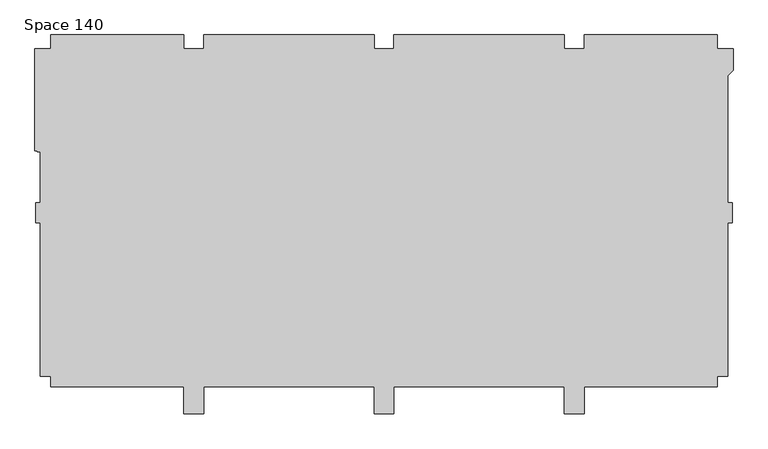
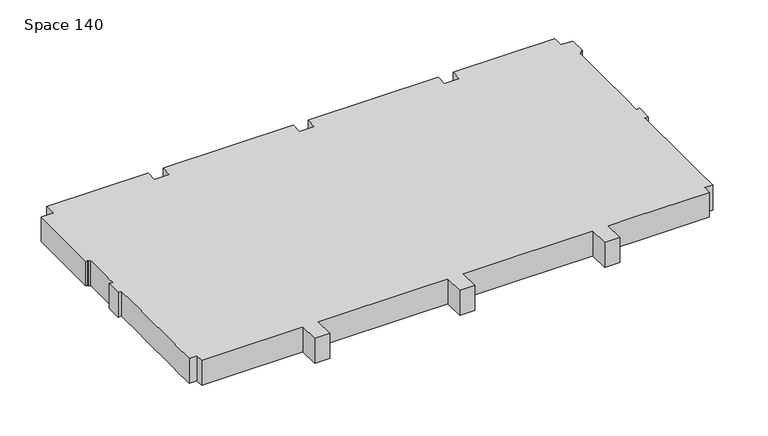
"""IFC4 building model written with IfcOpenShell, lengths in millimetres: proxy geometry, Space 140."""

from ifc_helpers import new_model, si_unit, origin, place, context, project, spatial, faceted_brep, source, transform, mapped, element, save


def space_140_8fd2c7b0(model_context):
    return source(origin(), model_context, "Body", "Brep", [
        faceted_brep([(-43930.8440345, 13392.940365, 3810.0), (-45315.1440345, 13392.940365, 3810.0), (-45315.1440345, 13392.940365, 6858.0), (-43930.8440345, 13392.940365, 6858.0), (-43930.8440345, 14624.840365, 3810.0), (-43930.8440345, 14624.840365, 6858.0), (-32221.4440345, 14624.840365, 3810.0), (-32221.4440345, 14624.840365, 6858.0), (-32221.4440345, 13392.940365, 3810.0), (-32221.4440345, 13392.940365, 6858.0), (-30468.8440345, 13392.940365, 3810.0), (-30468.8440345, 13392.940365, 6858.0), (-30468.8440345, 14624.840365, 3810.0), (-30468.8440345, 14624.840365, 6858.0), (-15457.4440345, 14624.840365, 3810.0), (-15457.4440345, 14624.840365, 6858.0), (-15457.4440345, 13392.940365, 3810.0), (-15457.4440345, 13392.940365, 6858.0), (-13704.8440345, 13392.940365, 3810.0), (-13704.8440345, 13392.940365, 6858.0), (-13704.8440345, 14624.840365, 3810.0), (-13704.8440345, 14624.840365, 6858.0), (1306.5559655, 14624.840365, 3810.0), (1306.5559655, 14624.840365, 6858.0), (1306.5559655, 13392.940365, 3810.0), (1306.5559655, 13392.940365, 6858.0), (3059.1559655, 13392.940365, 3810.0), (3059.1559655, 13392.940365, 6858.0), (3059.1559655, 14624.840365, 3810.0), (3059.1559655, 14624.840365, 6858.0), (14768.5559655, 14624.840365, 3810.0), (14768.5559655, 14624.840365, 6858.0), (14768.5559655, 13392.940365, 3810.0), (14768.5559655, 13392.940365, 6858.0), (16152.8559655, 13392.940365, 3810.0), (16152.8559655, 13392.940365, 6858.0), (16152.8559655, 11513.340365, 3810.0), (16152.8559655, 11513.340365, 6858.0), (15682.9559655, 11049.790365, 3810.0), (15682.9559655, 11049.790365, 6858.0), (15682.9559655, -145.259635, 3810.0), (15682.9559655, 623.090365, 3810.0), (15682.9559655, 991.390365, 3810.0), (15682.9559655, 7328.690365, 3810.0), (15682.9559655, 7696.990365, 3810.0), (15682.9559655, 10681.490365, 3810.0), (15682.9559655, 10681.490365, 6858.0), (15682.9559655, 7696.990365, 6858.0), (15682.9559655, 7328.690365, 6858.0), (15682.9559655, 991.390365, 6858.0), (15682.9559655, 623.090365, 6858.0), (15682.9559655, -145.259635, 6858.0), (16070.3059655, -145.259635, 3810.0), (16070.3059655, -145.259635, 6858.0), (16070.3059655, -1897.859635, 3810.0), (16070.3059655, -1897.859635, 6858.0), (15682.9559655, -1897.859635, 3810.0), (15682.9559655, -1897.859635, 6858.0), (15682.9559655, -15436.059635, 3810.0), (15682.9559655, -12788.109635, 3810.0), (15682.9559655, -12419.809635, 3810.0), (15682.9559655, -6082.509635, 3810.0), (15682.9559655, -5714.209635, 3810.0), (15682.9559655, -5714.209635, 6858.0), (15682.9559655, -6082.509635, 6858.0), (15682.9559655, -12419.809635, 6858.0), (15682.9559655, -12788.109635, 6858.0), (15682.9559655, -15436.059635, 6858.0), (14768.5559655, -15436.059635, 3810.0), (14768.5559655, -15436.059635, 6858.0), (14768.5559655, -16350.459635, 3810.0), (14768.5559655, -16350.459635, 6858.0), (3059.1559655, -16350.459635, 3810.0), (5903.9559655, -16350.459635, 3810.0), (5903.9559655, -16350.459635, 6858.0), (3059.1559655, -16350.459635, 6858.0), (3059.1559655, -18738.059635, 3810.0), (3059.1559655, -18738.059635, 6858.0), (1306.5559655, -18738.059635, 3810.0), (1306.5559655, -18738.059635, 6858.0), (1306.5559655, -16350.459635, 3810.0), (1306.5559655, -16350.459635, 6858.0), (-13704.8440345, -16350.459635, 3810.0), (-7659.6440345, -16350.459635, 3810.0), (-7659.6440345, -16350.459635, 6858.0), (-13704.8440345, -16350.459635, 6858.0), (-13704.8440345, -18738.059635, 3810.0), (-13704.8440345, -18738.059635, 6858.0), (-15457.4440345, -18738.059635, 3810.0), (-15457.4440345, -18738.059635, 6858.0), (-15457.4440345, -16350.459635, 3810.0), (-15457.4440345, -16350.459635, 6858.0), (-30468.8440345, -16350.459635, 3810.0), (-18810.2440345, -16350.459635, 3810.0), (-18810.2440345, -16350.459635, 6858.0), (-30468.8440345, -16350.459635, 6858.0), (-30468.8440345, -18738.059635, 3810.0), (-30468.8440345, -18738.059635, 6858.0), (-32221.4440345, -18738.059635, 3810.0), (-32221.4440345, -18738.059635, 6858.0), (-32221.4440345, -16350.459635, 3810.0), (-32221.4440345, -16350.459635, 6858.0), (-43930.8440345, -16350.459635, 3810.0), (-41498.7940345, -16350.459635, 3810.0), (-41498.7940345, -16350.459635, 6858.0), (-43930.8440345, -16350.459635, 6858.0), (-43930.8440345, -15436.059635, 3810.0), (-43930.8440345, -15436.059635, 6858.0), (-44845.2440345, -15436.059635, 3810.0), (-44845.2440345, -15436.059635, 6858.0), (-44845.2440345, -1897.859635, 3810.0), (-44845.2440345, -5714.209635, 3810.0), (-44845.2440345, -6082.509635, 3810.0), (-44845.2440345, -12419.809635, 3810.0), (-44845.2440345, -12788.109635, 3810.0), (-44845.2440345, -12788.109635, 6858.0), (-44845.2440345, -12419.809635, 6858.0), (-44845.2440345, -6082.509635, 6858.0), (-44845.2440345, -5714.209635, 6858.0), (-44845.2440345, -1897.859635, 6858.0), (-45232.5940345, -1897.859635, 3810.0), (-45232.5940345, -1897.859635, 6858.0), (-45232.5940345, -145.259635, 3810.0), (-45232.5940345, -145.259635, 6858.0), (-44845.2440345, -145.259635, 3810.0), (-44845.2440345, -145.259635, 6858.0), (-44845.2440345, 4344.190365, 3810.0), (-44845.2440345, 3975.890365, 3810.0), (-44845.2440345, 991.390365, 3810.0), (-44845.2440345, 623.090365, 3810.0), (-44845.2440345, 623.090365, 6858.0), (-44845.2440345, 991.390365, 6858.0), (-44845.2440345, 3975.890365, 6858.0), (-44845.2440345, 4344.190365, 6858.0), (-45092.8940345, 4344.190365, 3810.0), (-45092.8940345, 4344.190365, 6858.0), (-45092.8940345, 4433.090365, 3810.0), (-45092.8940345, 4433.090365, 6858.0), (-45315.1440345, 4433.090365, 3810.0), (-45315.1440345, 4433.090365, 6858.0)], [[[0, 1, 2, 3]], [[4, 0, 3, 5]], [[6, 4, 5, 7]], [[8, 6, 7, 9]], [[10, 8, 9, 11]], [[12, 10, 11, 13]], [[14, 12, 13, 15]], [[16, 14, 15, 17]], [[18, 16, 17, 19]], [[20, 18, 19, 21]], [[22, 20, 21, 23]], [[24, 22, 23, 25]], [[26, 24, 25, 27]], [[28, 26, 27, 29]], [[30, 28, 29, 31]], [[32, 30, 31, 33]], [[34, 32, 33, 35]], [[36, 34, 35, 37]], [[38, 36, 37, 39]], [[40, 41, 42, 43, 44, 45, 38, 39, 46, 47, 48, 49, 50, 51]], [[52, 40, 51, 53]], [[54, 52, 53, 55]], [[56, 54, 55, 57]], [[58, 59, 60, 61, 62, 56, 57, 63, 64, 65, 66, 67]], [[68, 58, 67, 69]], [[70, 68, 69, 71]], [[72, 73, 70, 71, 74, 75]], [[76, 72, 75, 77]], [[78, 76, 77, 79]], [[80, 78, 79, 81]], [[82, 83, 80, 81, 84, 85]], [[86, 82, 85, 87]], [[88, 86, 87, 89]], [[90, 88, 89, 91]], [[92, 93, 90, 91, 94, 95]], [[96, 92, 95, 97]], [[98, 96, 97, 99]], [[100, 98, 99, 101]], [[102, 103, 100, 101, 104, 105]], [[106, 102, 105, 107]], [[108, 106, 107, 109]], [[110, 111, 112, 113, 114, 108, 109, 115, 116, 117, 118, 119]], [[120, 110, 119, 121]], [[122, 120, 121, 123]], [[124, 122, 123, 125]], [[126, 127, 128, 129, 124, 125, 130, 131, 132, 133]], [[134, 126, 133, 135]], [[136, 134, 135, 137]], [[138, 136, 137, 139]], [[1, 138, 139, 2]], [[2, 139, 137, 135, 133, 132, 131, 130, 125, 123, 121, 119, 118, 117, 116, 115, 109, 107, 105, 104, 101, 99, 97, 95, 94, 91, 89, 87, 85, 84, 81, 79, 77, 75, 74, 71, 69, 67, 66, 65, 64, 63, 57, 55, 53, 51, 50, 49, 48, 47, 46, 39, 37, 35, 33, 31, 29, 27, 25, 23, 21, 19, 17, 15, 13, 11, 9, 7, 5, 3]], [[138, 1, 0, 4, 6, 8, 10, 12, 14, 16, 18, 20, 22, 24, 26, 28, 30, 32, 34, 36, 38, 45, 44, 43, 42, 41, 40, 52, 54, 56, 62, 61, 60, 59, 58, 68, 70, 73, 72, 76, 78, 80, 83, 82, 86, 88, 90, 93, 92, 96, 98, 100, 103, 102, 106, 108, 114, 113, 112, 111, 110, 120, 122, 124, 129, 128, 127, 126, 134, 136]]]),
    ])


if __name__ == "__main__":
    model = new_model("IFC4")
    model_context = context("Model", 3, world=origin())
    ifc_project = project(units=[si_unit("LENGTHUNIT", "METRE", prefix="MILLI")], contexts=[model_context])
    site = spatial("IfcSite", under=ifc_project)
    building = spatial("IfcBuilding", under=site)
    placement = place(None, origin())
    space_140_shape = space_140_8fd2c7b0(model_context)
    element("IfcBuildingElementProxy", 1, Name="Space 140", ObjectType="Space 140", at=placement, inside=building, context=model_context, shape_type="MappedRepresentation", body=[
        mapped(space_140_shape, transform((0.0, 0.0, 0.0), x_axis=(1.0, 0.0, 0.0), y_axis=(0.0, 1.0, 0.0), z_axis=(0.0, 0.0, 1.0))),
    ])
    save(model, "model.ifc")

# Revit data of these elements
# Element 1 (IfcBuildingElementProxy, "Space 140")
#   Materials on its faces: "Render Material 255-255-255"
# Materials
#   "Render Material 255-255-255": class "Unassigned", colour RGB 255 255 255, transparency 0
